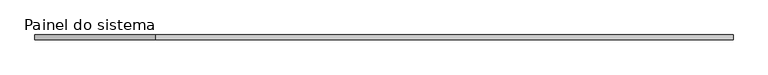
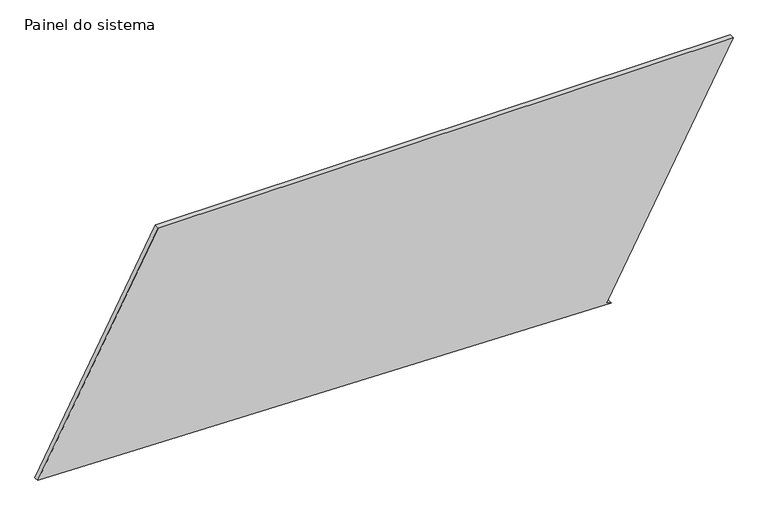
"""IFC4 building model written with IfcOpenShell, lengths in millimetres: plate geometry, Painel do sistema : Envidraçado."""

from ifc_helpers import new_model, si_unit, frame, origin, place, context, project, spatial, polyline, outline, extrude, source, transform, mapped, element, save


def painel_do_sistema_7dc68a2d(model_context):
    return source(origin(), model_context, "Body", "SweptSolid", [
        extrude(outline(polyline([(0.0, 1135.2774063), (11.7958757, 1113.2352349), (1196.9988874, 1747.4970389), (1196.9988874, -1141.9970515), (65.5411767, -1747.4970389), (0.0, 1135.2774063)])), frame((0.0, 24.5, 0.0), z_axis=(0.0, 1.0, 0.0), x_axis=(0.0, 0.0, 1.0)), (0.0, 0.0, 1.0), 25.0),
    ])


if __name__ == "__main__":
    model = new_model("IFC4")
    model_context = context("Model", 3, world=origin())
    ifc_project = project(units=[si_unit("LENGTHUNIT", "METRE", prefix="MILLI")], contexts=[model_context])
    site = spatial("IfcSite", under=ifc_project)
    building = spatial("IfcBuilding", under=site)
    placement = place(None, origin())
    painel_do_sistema_shape = painel_do_sistema_7dc68a2d(model_context)
    element("IfcPlate", 1, ObjectType="Painel do sistema : Envidraçado", at=placement, inside=building, context=model_context, shape_type="MappedRepresentation", body=[
        mapped(painel_do_sistema_shape, transform((0.0, 0.0, 0.0), x_axis=(1.0, 0.0, 0.0), y_axis=(0.0, 1.0, 0.0), z_axis=(0.0, 0.0, 1.0))),
    ])
    save(model, "model.ifc")

# Revit data of these elements
# Type "Painel do sistema : Envidraçado"
#   Construction Type Id = "GSP4R"
#   Analytic Construction = "Vidraça única Pilkington 1/8 pol"
#   Visual Light Transmittance = 0.9
#   Solar Heat Gain Coefficient = 0.86
#   Heat Transfer Coefficient (U) = 6.7069 W/(m²·K)
# Element 1 (IfcPlate, "Painel do sistema : Envidraçado")
#   Materials on its faces: "Vidro"
# Materials
#   "Vidro": class "Vidro", colour RGB 0 128 192, transparency 0.9, Description = "Vidro de sílica", Cost = 0
